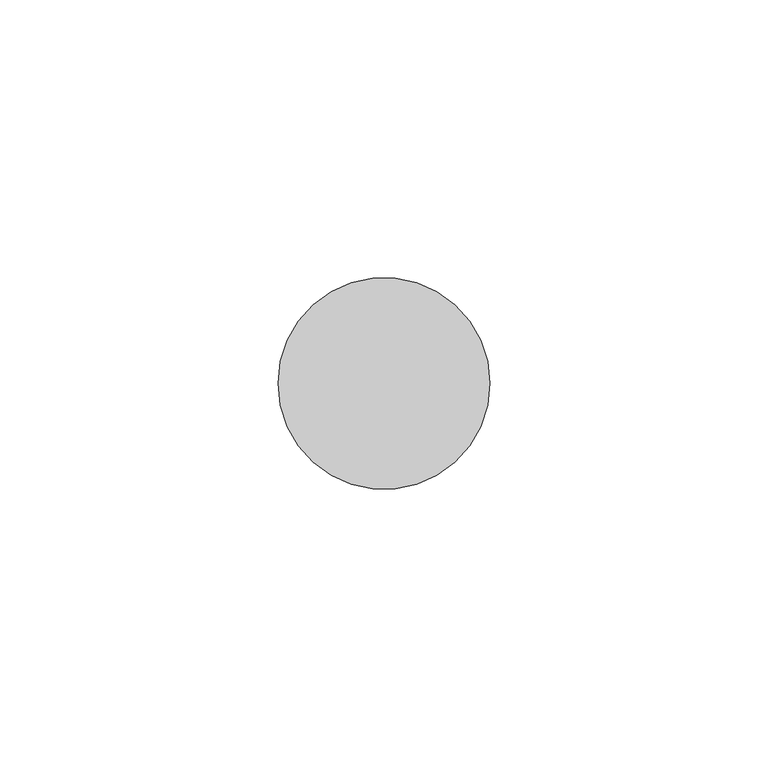
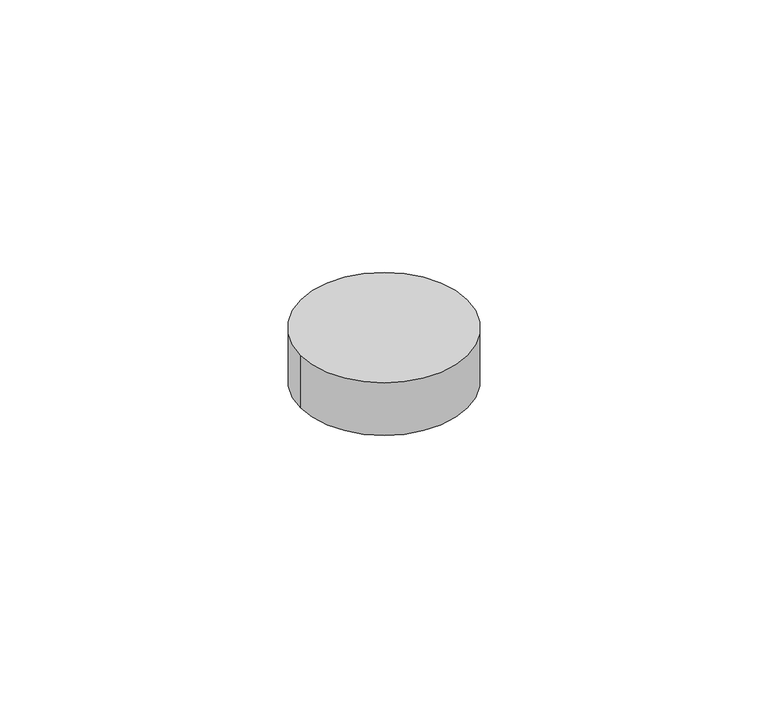
"""IFC4 building model written with IfcOpenShell, lengths in millimetres: proxy geometry, Bolt32:Bolt002:307957 : Bolt32:Bolt002:307957."""

import ifcopenshell
import ifcopenshell.guid

model = None  # the IFC model being written
_history = None  # IfcOwnerHistory: only IFC2X3 demands one
_inside = {}  # id of a spatial element -> (the spatial element, [elements in it])
_under = {}  # id of a project, library or spatial element -> (it, [spatial elements below it])
_declared = {}  # id of a project -> (the project, [libraries it declares])
_typed = {}  # id of a type object -> (the type object, [elements of that type])
_made_of = {}  # id of a material, layer set ... -> (it, [elements and type objects made of it])


def new_model(schema):
    """Start an empty IFC model of exactly this schema.

    Asked for "IFC4X3", IfcOpenShell would pick the latest addendum, in which some entities
    have other attributes; the version numbers below select the first issue.
    IFC2X3 requires an IfcOwnerHistory on every rooted entity: one is made here for all.
    """
    global model, _history
    if schema == "IFC4X3":
        model = ifcopenshell.file(schema_version=(4, 3, 0, 0))
    else:
        model = ifcopenshell.file(schema=schema)
    _inside.clear()
    _under.clear()
    _declared.clear()
    _typed.clear()
    _made_of.clear()
    _history = None
    if model.schema == "IFC2X3":
        org = make("IfcOrganization", Name="unknown")
        user = make(
            "IfcPersonAndOrganization",
            ThePerson=make("IfcPerson", FamilyName="unknown"),
            TheOrganization=org,
        )
        app = make(
            "IfcApplication",
            ApplicationDeveloper=org,
            Version="unknown",
            ApplicationFullName="unknown",
            ApplicationIdentifier="unknown",
        )
        _history = make(
            "IfcOwnerHistory",
            OwningUser=user,
            OwningApplication=app,
            ChangeAction="ADDED",
            CreationDate=0,
        )
    return model


def make(cls, **values):
    """One entity of the class cls with the attributes given. An attribute that is None is left unset."""
    return model.create_entity(
        cls, **{name: value for name, value in values.items() if value is not None}
    )


def rooted(cls, **values):
    """An entity with a GlobalId (a new one), such as an element, a storey or a relation."""
    return make(cls, GlobalId=ifcopenshell.guid.new(), OwnerHistory=_history, **values)


def si_unit(unit_type, name, prefix=None):
    """IfcSIUnit, for example si_unit("LENGTHUNIT", "METRE", prefix="MILLI")."""
    return make("IfcSIUnit", UnitType=unit_type, Prefix=prefix, Name=name)


def assignment(units):
    """IfcUnitAssignment: the units of a project."""
    return None if units is None else make("IfcUnitAssignment", Units=units)


def point(xyz):
    """IfcCartesianPoint."""
    return None if xyz is None else make("IfcCartesianPoint", Coordinates=xyz)


def direction(xyz):
    """IfcDirection."""
    return None if xyz is None else make("IfcDirection", DirectionRatios=xyz)


def frame(location, z_axis=None, x_axis=None):
    """IfcAxis2Placement3D, a coordinate frame: its origin and axes. An axis left out is left unset."""
    return make(
        "IfcAxis2Placement3D",
        Location=point(location),
        Axis=direction(z_axis),
        RefDirection=direction(x_axis),
    )


def frame_2d(location, x_axis=None):
    """IfcAxis2Placement2D, a coordinate frame in the plane: its origin and x axis."""
    return make(
        "IfcAxis2Placement2D", Location=point(location), RefDirection=direction(x_axis)
    )


def origin():
    """The frame at (0, 0, 0) with its axes left unset."""
    return frame((0.0, 0.0, 0.0))


def place(relative_to, where):
    """IfcLocalPlacement: puts the frame where relative to a parent placement (None: the world)."""
    return make(
        "IfcLocalPlacement", PlacementRelTo=relative_to, RelativePlacement=where
    )


def context(
    kind, dimensions, precision=None, world=None, true_north=None, identifier=None
):
    """IfcGeometricRepresentationContext, for example the 3D "Model" context."""
    return make(
        "IfcGeometricRepresentationContext",
        ContextIdentifier=identifier,
        ContextType=kind,
        CoordinateSpaceDimension=dimensions,
        Precision=precision,
        WorldCoordinateSystem=world,
        TrueNorth=true_north,
    )


def project(units=None, contexts=None):
    """IfcProject with its units and contexts."""
    return rooted(
        "IfcProject",
        Name="project",
        RepresentationContexts=contexts,
        UnitsInContext=assignment(units),
    )


def spatial(cls, under=None, at=None, **own):
    """A site, building, storey or space (cls), placed at a placement, below another one or the project."""
    s = rooted(cls, ObjectPlacement=at, **own)
    if under is not None:
        _under.setdefault(under.id(), (under, []))[1].append(s)
    return s


def circle_curve(where, radius):
    """IfcCircle in the frame where."""
    return make("IfcCircle", Position=where, Radius=radius)


def trimmed(basis, trim1, trim2, sense, master):
    """IfcTrimmedCurve: the piece of a basis curve between two trims."""
    return make(
        "IfcTrimmedCurve",
        BasisCurve=basis,
        Trim1=trim1,
        Trim2=trim2,
        SenseAgreement=sense,
        MasterRepresentation=master,
    )


def segment(curve, same_sense, transition):
    """IfcCompositeCurveSegment."""
    return make(
        "IfcCompositeCurveSegment",
        Transition=transition,
        SameSense=same_sense,
        ParentCurve=curve,
    )


def composite_curve(segments, self_intersect=None):
    """IfcCompositeCurve: segments joined end to end."""
    return make("IfcCompositeCurve", Segments=segments, SelfIntersect=self_intersect)


def outline(outer, holes=None, kind="AREA"):
    """IfcArbitraryClosedProfileDef: a profile drawn as a closed curve; with holes, ...WithVoids."""
    if holes is None:
        return make("IfcArbitraryClosedProfileDef", ProfileType=kind, OuterCurve=outer)
    return make(
        "IfcArbitraryProfileDefWithVoids",
        ProfileType=kind,
        OuterCurve=outer,
        InnerCurves=holes,
    )


def extrude(swept, where, along, depth):
    """IfcExtrudedAreaSolid: the profile swept, set in the frame where, extruded along a direction by depth."""
    return make(
        "IfcExtrudedAreaSolid",
        SweptArea=swept,
        Position=where,
        ExtrudedDirection=direction(along),
        Depth=depth,
    )


def shape(context_of_items, identifier, shape_type, items):
    """IfcShapeRepresentation: the items that make up one representation, for example the "Body"."""
    return make(
        "IfcShapeRepresentation",
        ContextOfItems=context_of_items,
        RepresentationIdentifier=identifier,
        RepresentationType=shape_type,
        Items=items,
    )


def source(mapping_origin, context_of_items, identifier, shape_type, items):
    """IfcRepresentationMap: a shape defined once, which mapped items show again and again."""
    return make(
        "IfcRepresentationMap",
        MappingOrigin=mapping_origin,
        MappedRepresentation=shape(context_of_items, identifier, shape_type, items),
    )


def transform(
    local_origin,
    x_axis=None,
    y_axis=None,
    z_axis=None,
    scale=None,
    scale2=None,
    scale3=None,
    uniform=True,
):
    """IfcCartesianTransformationOperator3D, or its non-uniform kind. x_axis, y_axis, z_axis: its Axis1, 2, 3."""
    if uniform:
        return make(
            "IfcCartesianTransformationOperator3D",
            Axis1=direction(x_axis),
            Axis2=direction(y_axis),
            LocalOrigin=point(local_origin),
            Scale=scale,
            Axis3=direction(z_axis),
        )
    return make(
        "IfcCartesianTransformationOperator3DnonUniform",
        Axis1=direction(x_axis),
        Axis2=direction(y_axis),
        LocalOrigin=point(local_origin),
        Scale=scale,
        Axis3=direction(z_axis),
        Scale2=scale2,
        Scale3=scale3,
    )


def mapped(mapping_source, mapping_target):
    """IfcMappedItem: shows the shape of a source again, moved by a transform."""
    return make(
        "IfcMappedItem", MappingSource=mapping_source, MappingTarget=mapping_target
    )


def made_of(thing, what):
    """Note that an element or type object is made of a material, layer set ...; save() writes the relation."""
    if what is not None:
        _made_of.setdefault(what.id(), (what, []))[1].append(thing)
    return thing


def element(
    cls,
    number,
    at=None,
    inside=None,
    cuts=None,
    type_object=None,
    material=None,
    context=None,
    identifier="Body",
    shape_type=None,
    held_by="IfcProductDefinitionShape",
    body=None,
    shapes=None,
    **own,
):
    """One element of the class cls, such as IfcWall. Its Tag is "e" and its number.

    at: its placement. inside: the storey or other place that contains it. cuts: it is an
    opening in that element (IfcRelVoidsElement). A single representation is given by context,
    identifier, shape_type and body (its items); several are given by shapes. held_by: the class
    of the entity that holds the representations. save() writes the other relations.
    """
    e = rooted(cls, Tag="e%d" % number, ObjectPlacement=at, **own)
    if body is not None:
        shapes = [shape(context, identifier, shape_type, body)]
    if shapes is not None:
        e.Representation = make(held_by, Representations=shapes)
    if inside is not None:
        _inside.setdefault(inside.id(), (inside, []))[1].append(e)
    if cuts is not None:
        rooted(
            "IfcRelVoidsElement", RelatingBuildingElement=cuts, RelatedOpeningElement=e
        )
    if type_object is not None:
        _typed.setdefault(type_object.id(), (type_object, []))[1].append(e)
    return made_of(e, material)


def aggregate(whole, parts):
    """IfcRelAggregates: a whole, such as a stair, and the parts it consists of."""
    return rooted("IfcRelAggregates", RelatingObject=whole, RelatedObjects=parts)


def save(model, path):
    """Write the relations noted so far, then the file.

    IfcRelAggregates (storeys below a building ...), IfcRelContainedInSpatialStructure (elements
    in a storey), IfcRelDefinesByType, IfcRelAssociatesMaterial and IfcRelDeclares: one each for
    every whole, place, type object, material and project.
    """
    for whole, parts in _under.values():
        aggregate(whole, parts)
    for where, things in _inside.values():
        rooted(
            "IfcRelContainedInSpatialStructure",
            RelatedElements=things,
            RelatingStructure=where,
        )
    for kind, things in _typed.values():
        rooted("IfcRelDefinesByType", RelatedObjects=things, RelatingType=kind)
    for what, things in _made_of.values():
        rooted("IfcRelAssociatesMaterial", RelatedObjects=things, RelatingMaterial=what)
    for by, libraries in _declared.values():
        rooted("IfcRelDeclares", RelatingContext=by, RelatedDefinitions=libraries)
    model.write(path)


def generic_models_1788a601(model_context):
    return source(origin(), model_context, "Body", "SweptSolid", [
        extrude(outline(composite_curve([segment(trimmed(circle_curve(frame_2d((12192.2703385, -1503.5124296)), 19.05), [point((12173.2203385, -1503.5124296))], [point((12211.3203385, -1503.5124296))], False, "CARTESIAN"), True, "CONTINUOUS"), segment(trimmed(circle_curve(frame_2d((12192.2703385, -1503.5124296)), 19.05), [point((12211.3203385, -1503.5124296))], [point((12173.2203385, -1503.5124296))], False, "CARTESIAN"), True, "CONTINUOUS")], self_intersect=False)), frame((0.0, 0.0, 40008.048), z_axis=(0.0, 0.0, 1.0), x_axis=(1.0, 0.0, 0.0)), (0.0, 0.0, 1.0), 12.7),
    ])


if __name__ == "__main__":
    model = new_model("IFC4")
    model_context = context("Model", 3, world=origin())
    ifc_project = project(units=[si_unit("LENGTHUNIT", "METRE", prefix="MILLI")], contexts=[model_context])
    site = spatial("IfcSite", under=ifc_project)
    building = spatial("IfcBuilding", under=site)
    placement = place(None, origin())
    generic_models_shape = generic_models_1788a601(model_context)
    element("IfcBuildingElementProxy", 1, Name="Bolt32:Bolt002:307957 : Bolt32:Bolt002:307957", ObjectType="Bolt32:Bolt002:307957 : Bolt32:Bolt002:307957", at=placement, inside=building, context=model_context, shape_type="MappedRepresentation", body=[
        mapped(generic_models_shape, transform((0.0, 0.0, 0.0), x_axis=(1.0, 0.0, 0.0), y_axis=(0.0, 1.0, 0.0), z_axis=(0.0, 0.0, 1.0))),
    ])
    save(model, "model.ifc")

# Revit data of these elements
# Type "Bolt32:Bolt002:307957 : Bolt32:Bolt002:307957"
#   NameOverride = "Bolt32:Bolt002:307957"
#   ObjectTypeOverride = "Bolt32:Bolt002"
#   Reference = "Bolt002"
#   Category = "Generic Models"
#   Tag = "307957"
# Element 1 (IfcBuildingElementProxy, "Bolt32:Bolt002:307957 : Bolt32:Bolt002:307957")
#   Materials on its faces: "BOLTS CONCEALED BY FLOOR FINISH"
# Materials
#   "BOLTS CONCEALED BY FLOOR FINISH": class "Unassigned", colour RGB 128 128 128, transparency 0
